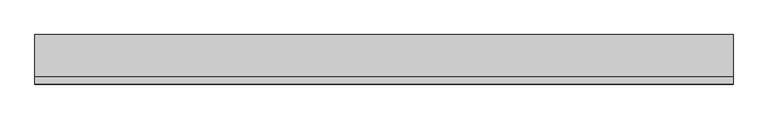
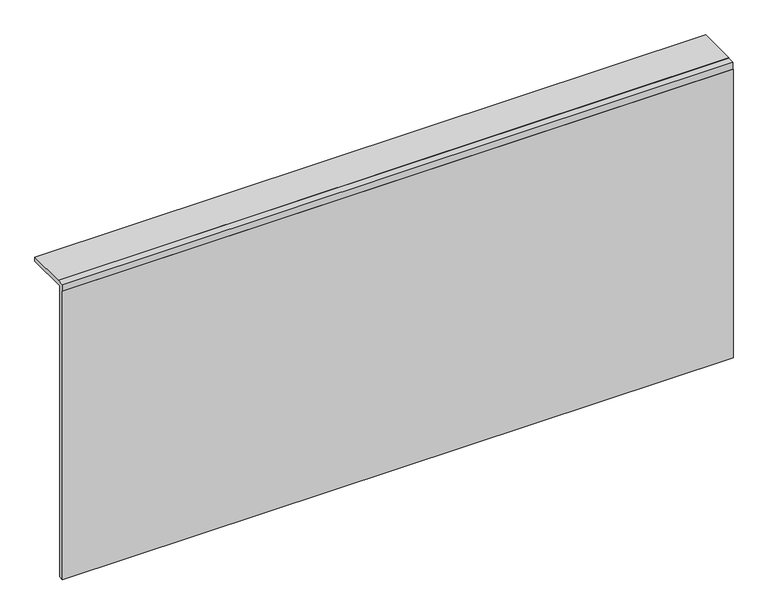
"""IFC4 building model written with IfcOpenShell, lengths in millimetres: proxy geometry, Gypsum014 1659 : Gypsum014 1659."""

from ifc_helpers import new_model, si_unit, frame, origin, place, context, project, spatial, polyline, outline, extrude, source, transform, mapped, element, save


def generic_models_078ccaee(model_context):
    return source(origin(), model_context, "Body", "SweptSolid", [
        extrude(outline(polyline([(9576.3500834, 36582.096), (9576.3500834, 37490.9066598), (9577.6300834, 37490.9066598), (9577.6300834, 37512.0598438), (9598.7832673, 37512.0598438), (9598.7832673, 37513.3398438), (9718.4918386, 37513.3398438), (9718.4918386, 37500.1015625), (9590.6383229, 37500.1015625), (9590.6383229, 36582.096), (9576.3500834, 36582.096)])), frame((3694.2883192, 0.0, 0.0), z_axis=(1.0, 0.0, 0.0), x_axis=(0.0, 1.0, 0.0)), (0.0, 0.0, 1.0), 2000.0),
    ])


if __name__ == "__main__":
    model = new_model("IFC4")
    model_context = context("Model", 3, world=origin())
    ifc_project = project(units=[si_unit("LENGTHUNIT", "METRE", prefix="MILLI")], contexts=[model_context])
    site = spatial("IfcSite", under=ifc_project)
    building = spatial("IfcBuilding", under=site)
    placement = place(None, origin())
    generic_models_shape = generic_models_078ccaee(model_context)
    element("IfcBuildingElementProxy", 1, Name="Gypsum014 1659 : Gypsum014 1659", ObjectType="Gypsum014 1659 : Gypsum014 1659", at=placement, inside=building, context=model_context, shape_type="MappedRepresentation", body=[
        mapped(generic_models_shape, transform((0.0, 0.0, 0.0), x_axis=(1.0, 0.0, 0.0), y_axis=(0.0, 1.0, 0.0), z_axis=(0.0, 0.0, 1.0))),
    ])
    save(model, "model.ifc")

# Revit data of these elements
# Type "Gypsum014 1659 : Gypsum014 1659"
#   NameOverride = "Gypsum014"
# Element 1 (IfcBuildingElementProxy, "Gypsum014 1659 : Gypsum014 1659")
#   Materials on its faces: "5/8\"  GYPSUM BOARD"
# Materials
#   "5/8\"  GYPSUM BOARD": class "Unassigned", colour RGB 255 255 255, transparency 0, Cost = 0
